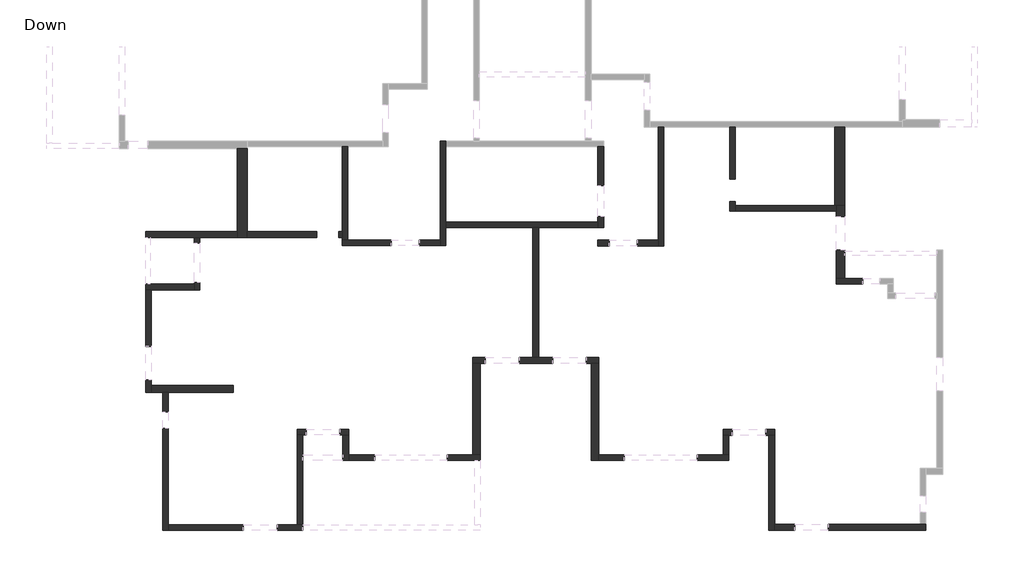
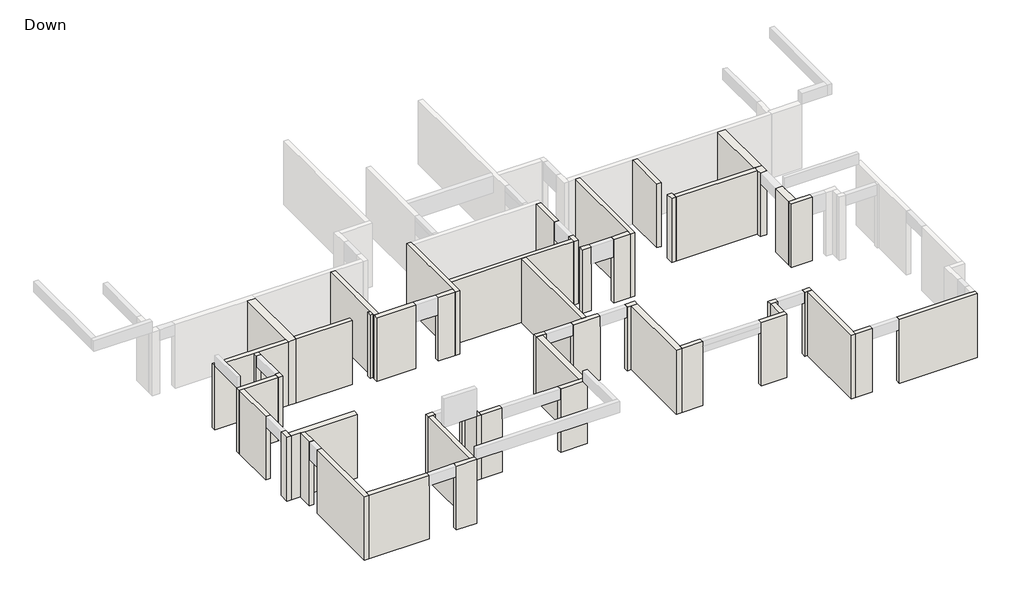
# One storey, part 1 of 3: 51 walls.
"""IFC4 building model written with IfcOpenShell, lengths in millimetres."""

from ifc_helpers import new_model, si_unit, origin, place, context, project, spatial, faceted_brep, element, save

model = new_model("IFC4")

# Units and contexts
model_context = context("Model", 3, world=origin())
ifc_project = project(units=[si_unit("LENGTHUNIT", "METRE", prefix="MILLI")], contexts=[model_context])

# Site, building, storey
site = spatial("IfcSite", under=ifc_project)
building = spatial("IfcBuilding", under=site)
storey = spatial("IfcBuildingStorey", under=building, Name="Down", Elevation=0.0)

# Walls
placement = place(None, origin())
element("IfcWall", 1, ObjectType="20", at=placement, inside=storey, context=model_context, shape_type="Brep", body=[
    faceted_brep([(-6090.9338154, -2994.7427075, 0.0), (-9365.9338154, -2994.7427075, 0.0), (-9365.9338154, -2994.7427075, 3000.0), (-6090.9338154, -2994.7427075, 3000.0), (-6090.9338154, -3194.7427075, 0.0), (-6090.9338154, -3194.7427075, 3000.0), (-7434.594706, -3194.7427075, 3000.0), (-7634.594706, -3194.7427075, 3000.0), (-9365.9338154, -3194.7427075, 3000.0), (-9365.9338154, -3194.7427075, 2780.0), (-9365.9338154, -3194.7427075, 0.0), (-7634.594706, -3194.7427075, 0.0), (-7434.594706, -3194.7427075, 0.0)], [[[0, 1, 2, 3]], [[4, 5, 6, 7, 8, 9, 10, 11, 12]], [[1, 0, 4, 12, 11, 10]], [[2, 1, 10, 9, 8]], [[3, 2, 8, 7, 6, 5]], [[0, 3, 5, 4]]]),
])
element("IfcWall", 2, ObjectType="20", at=placement, inside=storey, context=model_context, shape_type="Brep", body=[
    faceted_brep([(-7634.594706, -3194.7427075, 0.0), (-7634.594706, -3392.9835498, 0.0), (-7634.594706, -3392.9835498, 2500.0), (-7634.594706, -3392.9835498, 3000.0), (-7634.594706, -3194.7427075, 3000.0), (-7434.594706, -3194.7427075, 0.0), (-7434.594706, -3194.7427075, 2780.0), (-7434.594706, -3194.7427075, 3000.0), (-7434.594706, -3392.9835498, 3000.0), (-7434.594706, -3392.9835498, 2500.0), (-7434.594706, -3392.9835498, 0.0)], [[[0, 1, 2, 3, 4]], [[5, 6, 7, 8, 9, 10]], [[1, 0, 5, 10]], [[3, 2, 1, 10, 9, 8]], [[4, 3, 8, 7]], [[0, 4, 7, 6, 5]]]),
])
element("IfcWall", 3, ObjectType="20", at=placement, inside=storey, context=model_context, shape_type="Brep", body=[
    faceted_brep([(-5740.9338154, -3194.7427075, 0.0), (-3252.010806, -3194.7427075, 0.0), (-3252.010806, -3194.7427075, 2780.0), (-3252.010806, -3194.7427075, 3000.0), (-5740.9338154, -3194.7427075, 3000.0), (-5740.9338154, -2994.7427075, 0.0), (-5740.9338154, -2994.7427075, 2780.0), (-5740.9338154, -2994.7427075, 3000.0), (-3252.010806, -2994.7427075, 3000.0), (-3252.010806, -2994.7427075, 2780.0), (-3252.010806, -2994.7427075, 0.0)], [[[0, 1, 2, 3, 4]], [[5, 6, 7, 8, 9, 10]], [[1, 0, 5, 10]], [[3, 2, 1, 10, 9, 8]], [[4, 3, 8, 7]], [[0, 4, 7, 6, 5]]]),
])
element("IfcWall", 4, ObjectType="20", at=placement, inside=storey, context=model_context, shape_type="Brep", body=[
    faceted_brep([(-2456.1345173, -3194.0144776, 0.0), (-2336.5139865, -3194.0144776, 0.0), (-2336.5139865, -3194.0144776, 2780.0), (-2336.5139865, -3194.0144776, 3000.0), (-2456.1345173, -3194.0144776, 3000.0), (-2456.1345173, -3194.0144776, 2780.0), (-2456.1345173, -2994.0144776, 0.0), (-2456.1345173, -2994.0144776, 2780.0), (-2456.1345173, -2994.0144776, 3000.0), (-2336.5139865, -2994.0144776, 3000.0), (-2336.5139865, -2994.0144776, 2780.0), (-2336.5139865, -2994.0144776, 0.0), (-2456.1345173, -2994.7427075, 3000.0)], [[[0, 1, 2, 3, 4, 5]], [[6, 7, 8, 9, 10, 11]], [[1, 0, 6, 11]], [[4, 3, 9, 8, 12]], [[0, 5, 4, 12, 8, 7, 6]], [[3, 2, 1, 11, 10, 9]]]),
])
element("IfcWall", 5, ObjectType="20", at=placement, inside=storey, context=model_context, shape_type="Brep", body=[
    faceted_brep([(-2336.5139865, -3494.0144776, 0.0), (-591.3286388, -3494.0144776, 0.0), (-591.3286388, -3494.0144776, 2180.0), (-591.3286388, -3494.0144776, 3000.0), (-2336.5139865, -3494.0144776, 3000.0), (-2336.5139865, -3494.0144776, 2780.0), (-2336.5139865, -3294.0144776, 0.0), (-2336.5139865, -3294.0144776, 3000.0), (-2136.5139865, -3294.0144776, 3000.0), (-591.3286388, -3294.0144776, 3000.0), (-591.3286388, -3294.0144776, 2180.0), (-591.3286388, -3294.0144776, 0.0), (-2136.5139865, -3294.0144776, 0.0)], [[[0, 1, 2, 3, 4, 5]], [[6, 7, 8, 9, 10, 11, 12]], [[1, 0, 6, 12, 11]], [[3, 2, 1, 11, 10, 9]], [[4, 3, 9, 8, 7]], [[0, 5, 4, 7, 6]]]),
])
element("IfcWall", 6, ObjectType="20", at=placement, inside=storey, context=model_context, shape_type="Brep", body=[
    faceted_brep([(-2136.5139865, -3294.0144776, 0.0), (-2136.5139865, 51.1884177, 0.0), (-2136.5139865, 51.1884177, 2780.0), (-2136.5139865, 51.1884177, 3000.0), (-2136.5139865, -3294.0144776, 3000.0), (-2136.5139865, -3294.0144776, 2780.0), (-2336.5139865, -3294.0144776, 0.0), (-2336.5139865, -3294.0144776, 3000.0), (-2336.5139865, -3194.0144776, 3000.0), (-2336.5139865, -2994.0144776, 3000.0), (-2336.5139865, 51.1884177, 3000.0), (-2336.5139865, 51.1884177, 2780.0), (-2336.5139865, 51.1884177, 0.0), (-2336.5139865, -2994.0144776, 0.0), (-2336.5139865, -3194.0144776, 0.0)], [[[0, 1, 2, 3, 4, 5]], [[6, 7, 8, 9, 10, 11, 12, 13, 14]], [[1, 0, 6, 14, 13, 12]], [[4, 3, 10, 9, 8, 7]], [[3, 2, 1, 12, 11, 10]], [[0, 5, 4, 7, 6]]]),
])
element("IfcWall", 7, ObjectType="20", at=placement, inside=storey, context=model_context, shape_type="Brep", body=[
    faceted_brep([(1160.820407, 252.3535615, 0.0), (1160.820407, -3294.0144776, 0.0), (1160.820407, -3494.0144776, 0.0), (1160.820407, -3494.0144776, 3000.0), (1160.820407, -3294.0144776, 3000.0), (1160.820407, 252.3535615, 3000.0), (1160.820407, 252.3535615, 2780.0), (1360.820407, 252.3535615, 0.0), (1360.820407, 252.3535615, 3000.0), (1360.820407, 52.3535615, 3000.0), (1360.820407, -2647.6464385, 3000.0), (1360.820407, -2847.6464385, 3000.0), (1360.820407, -3494.0144776, 3000.0), (1360.820407, -3494.0144776, 2780.0), (1360.820407, -3494.0144776, 0.0), (1360.820407, -2847.6464385, 0.0), (1360.820407, -2647.6464385, 0.0), (1360.820407, 52.3535615, 0.0)], [[[0, 1, 2, 3, 4, 5, 6]], [[7, 8, 9, 10, 11, 12, 13, 14, 15, 16, 17]], [[2, 1, 0, 7, 17, 16, 15, 14]], [[5, 4, 3, 12, 11, 10, 9, 8]], [[3, 2, 14, 13, 12]], [[0, 6, 5, 8, 7]]]),
])
element("IfcWall", 8, ObjectType="20", at=placement, inside=storey, context=model_context, shape_type="Brep", body=[
    faceted_brep([(1360.820407, -2847.6464385, 0.0), (4485.405294, -2847.6464385, 0.0), (4685.405294, -2847.6464385, 0.0), (6810.820407, -2847.6464385, 0.0), (6810.820407, -2847.6464385, 2780.0), (6810.820407, -2847.6464385, 3000.0), (4685.405294, -2847.6464385, 3000.0), (4485.405294, -2847.6464385, 3000.0), (1360.820407, -2847.6464385, 3000.0), (1360.820407, -2847.6464385, 2780.0), (1360.820407, -2647.6464385, 0.0), (1360.820407, -2647.6464385, 3000.0), (6810.820407, -2647.6464385, 3000.0), (6810.820407, -2647.6464385, 0.0)], [[[0, 1, 2, 3, 4, 5, 6, 7, 8, 9]], [[10, 11, 12, 13]], [[3, 2, 1, 0, 10, 13]], [[8, 7, 6, 5, 12, 11]], [[0, 9, 8, 11, 10]], [[5, 4, 3, 13, 12]]]),
])
element("IfcWall", 9, ObjectType="20", at=placement, inside=storey, context=model_context, shape_type="Brep", body=[
    faceted_brep([(7010.820407, -2847.6464385, 0.0), (7010.820407, -2447.6464385, 0.0), (7010.820407, -2447.6464385, 2180.0), (7010.820407, -2447.6464385, 3000.0), (7010.820407, -2847.6464385, 3000.0), (7010.820407, -2847.6464385, 2780.0), (6810.820407, -2847.6464385, 0.0), (6810.820407, -2847.6464385, 2780.0), (6810.820407, -2847.6464385, 3000.0), (6810.820407, -2647.6464385, 3000.0), (6810.820407, -2447.6464385, 3000.0), (6810.820407, -2447.6464385, 2180.0), (6810.820407, -2447.6464385, 0.0), (6810.820407, -2647.6464385, 0.0)], [[[0, 1, 2, 3, 4, 5]], [[6, 7, 8, 9, 10, 11, 12, 13]], [[1, 0, 6, 13, 12]], [[3, 2, 1, 12, 11, 10]], [[4, 3, 10, 9, 8]], [[0, 5, 4, 8, 7, 6]]]),
])
element("IfcWall", 10, ObjectType="20", at=placement, inside=storey, context=model_context, shape_type="Brep", body=[
    faceted_brep([(6810.820407, 52.3535615, 0.0), (6810.820407, -1347.6464385, 0.0), (6810.820407, -1347.6464385, 2180.0), (6810.820407, -1347.6464385, 3000.0), (6810.820407, 52.3535615, 3000.0), (7010.820407, 52.3535615, 0.0), (7010.820407, 52.3535615, 3000.0), (7010.820407, -1347.6464385, 3000.0), (7010.820407, -1347.6464385, 2180.0), (7010.820407, -1347.6464385, 0.0)], [[[0, 1, 2, 3, 4]], [[5, 6, 7, 8, 9]], [[1, 0, 5, 9]], [[3, 2, 1, 9, 8, 7]], [[4, 3, 7, 6]], [[0, 4, 6, 5]]]),
])
element("IfcWall", 11, ObjectType="20", at=placement, inside=storey, context=model_context, shape_type="Brep", body=[
    faceted_brep([(-7634.594706, -4812.9835498, 0.0), (-7634.594706, -4872.9835498, 0.0), (-7634.594706, -5072.9835498, 0.0), (-7634.594706, -5072.9835498, 3000.0), (-7634.594706, -4872.9835498, 3000.0), (-7634.594706, -4812.9835498, 3000.0), (-7634.594706, -4812.9835498, 2500.0), (-7434.594706, -4812.9835498, 0.0), (-7434.594706, -4812.9835498, 2500.0), (-7434.594706, -4812.9835498, 3000.0), (-7434.594706, -5072.9835498, 3000.0), (-7434.594706, -5072.9835498, 2780.0), (-7434.594706, -5072.9835498, 0.0)], [[[0, 1, 2, 3, 4, 5, 6]], [[7, 8, 9, 10, 11, 12]], [[2, 1, 0, 7, 12]], [[5, 4, 3, 10, 9]], [[0, 6, 5, 9, 8, 7]], [[3, 2, 12, 11, 10]]]),
])
element("IfcWall", 12, ObjectType="20", at=placement, inside=storey, context=model_context, shape_type="Brep", body=[
    faceted_brep([(-7634.594706, -4872.9835498, 0.0), (-9364.594706, -4872.9835498, 0.0), (-9364.594706, -4872.9835498, 3000.0), (-7634.594706, -4872.9835498, 3000.0), (-7634.594706, -4872.9835498, 2780.0), (-7634.594706, -5072.9835498, 0.0), (-7634.594706, -5072.9835498, 3000.0), (-9164.594706, -5072.9835498, 3000.0), (-9364.594706, -5072.9835498, 3000.0), (-9364.594706, -5072.9835498, 0.0), (-9164.594706, -5072.9835498, 0.0)], [[[0, 1, 2, 3, 4]], [[5, 6, 7, 8, 9, 10]], [[1, 0, 5, 10, 9]], [[3, 2, 8, 7, 6]], [[0, 4, 3, 6, 5]], [[2, 1, 9, 8]]]),
])
element("IfcWall", 13, ObjectType="20", at=placement, inside=storey, context=model_context, shape_type="Brep", body=[
    faceted_brep([(-9364.594706, -5072.9835498, 0.0), (-9364.594706, -7092.9835498, 0.0), (-9364.594706, -7092.9835498, 2500.0), (-9364.594706, -7092.9835498, 3000.0), (-9364.594706, -5072.9835498, 3000.0), (-9164.594706, -5072.9835498, 0.0), (-9164.594706, -5072.9835498, 2780.0), (-9164.594706, -5072.9835498, 3000.0), (-9164.594706, -7092.9835498, 3000.0), (-9164.594706, -7092.9835498, 2500.0), (-9164.594706, -7092.9835498, 0.0)], [[[0, 1, 2, 3, 4]], [[5, 6, 7, 8, 9, 10]], [[1, 0, 5, 10]], [[3, 2, 1, 10, 9, 8]], [[4, 3, 8, 7]], [[0, 4, 7, 6, 5]]]),
])
element("IfcWall", 14, ObjectType="20", at=placement, inside=storey, context=model_context, shape_type="Brep", body=[
    faceted_brep([(-9364.594706, -8292.9835498, 0.0), (-9364.594706, -8747.9835498, 0.0), (-9364.594706, -8747.9835498, 3000.0), (-9364.594706, -8292.9835498, 3000.0), (-9364.594706, -8292.9835498, 2500.0), (-9164.594706, -8292.9835498, 0.0), (-9164.594706, -8292.9835498, 2500.0), (-9164.594706, -8292.9835498, 3000.0), (-9164.594706, -8497.9835498, 3000.0), (-9164.594706, -8747.9835498, 3000.0), (-9164.594706, -8747.9835498, 0.0), (-9164.594706, -8497.9835498, 0.0)], [[[0, 1, 2, 3, 4]], [[5, 6, 7, 8, 9, 10, 11]], [[1, 0, 5, 11, 10]], [[3, 2, 9, 8, 7]], [[0, 4, 3, 7, 6, 5]], [[2, 1, 10, 9]]]),
])
element("IfcWall", 15, ObjectType="20", at=placement, inside=storey, context=model_context, shape_type="Brep", body=[
    faceted_brep([(-8764.594706, -8747.9835498, 0.0), (-8764.594706, -9442.9835498, 0.0), (-8764.594706, -9442.9835498, 2180.0), (-8764.594706, -9442.9835498, 3000.0), (-8764.594706, -8747.9835498, 3000.0), (-8564.594706, -8747.9835498, 0.0), (-8564.594706, -8747.9835498, 2780.0), (-8564.594706, -8747.9835498, 3000.0), (-8564.594706, -9442.9835498, 3000.0), (-8564.594706, -9442.9835498, 2180.0), (-8564.594706, -9442.9835498, 0.0)], [[[0, 1, 2, 3, 4]], [[5, 6, 7, 8, 9, 10]], [[1, 0, 5, 10]], [[3, 2, 1, 10, 9, 8]], [[4, 3, 8, 7]], [[0, 4, 7, 6, 5]]]),
])
element("IfcWall", 16, ObjectType="20", at=placement, inside=storey, context=model_context, shape_type="Brep", body=[
    faceted_brep([(-8764.594706, -10042.9835498, 0.0), (-8764.594706, -13682.9835498, 0.0), (-8764.594706, -13682.9835498, 3000.0), (-8764.594706, -10042.9835498, 3000.0), (-8764.594706, -10042.9835498, 2180.0), (-8564.594706, -10042.9835498, 0.0), (-8564.594706, -10042.9835498, 2180.0), (-8564.594706, -10042.9835498, 3000.0), (-8564.594706, -13482.9835498, 3000.0), (-8564.594706, -13682.9835498, 3000.0), (-8564.594706, -13682.9835498, 0.0), (-8564.594706, -13482.9835498, 0.0)], [[[0, 1, 2, 3, 4]], [[5, 6, 7, 8, 9, 10, 11]], [[1, 0, 5, 11, 10]], [[3, 2, 9, 8, 7]], [[0, 4, 3, 7, 6, 5]], [[2, 1, 10, 9]]]),
])
element("IfcWall", 17, ObjectType="20", at=placement, inside=storey, context=model_context, shape_type="Brep", body=[
    faceted_brep([(-8564.594706, -13682.9835498, 0.0), (-5884.594706, -13682.9835498, 0.0), (-5884.594706, -13682.9835498, 2500.0), (-5884.594706, -13682.9835498, 3000.0), (-8564.594706, -13682.9835498, 3000.0), (-8564.594706, -13482.9835498, 0.0), (-8564.594706, -13482.9835498, 2780.0), (-8564.594706, -13482.9835498, 3000.0), (-5884.594706, -13482.9835498, 3000.0), (-5884.594706, -13482.9835498, 2500.0), (-5884.594706, -13482.9835498, 0.0)], [[[0, 1, 2, 3, 4]], [[5, 6, 7, 8, 9, 10]], [[1, 0, 5, 10]], [[3, 2, 1, 10, 9, 8]], [[4, 3, 8, 7]], [[0, 4, 7, 6, 5]]]),
])
element("IfcWall", 18, ObjectType="20", at=placement, inside=storey, context=model_context, shape_type="Brep", body=[
    faceted_brep([(-4664.594706, -13682.9835498, 0.0), (-3754.594706, -13682.9835498, 0.0), (-3754.594706, -13682.9835498, 3000.0), (-4664.594706, -13682.9835498, 3000.0), (-4664.594706, -13682.9835498, 2500.0), (-4664.594706, -13482.9835498, 0.0), (-4664.594706, -13482.9835498, 2500.0), (-4664.594706, -13482.9835498, 3000.0), (-3954.594706, -13482.9835498, 3000.0), (-3754.594706, -13482.9835498, 3000.0), (-3754.594706, -13482.9835498, 0.0), (-3954.594706, -13482.9835498, 0.0)], [[[0, 1, 2, 3, 4]], [[5, 6, 7, 8, 9, 10, 11]], [[1, 0, 5, 11, 10]], [[3, 2, 9, 8, 7]], [[0, 4, 3, 7, 6, 5]], [[2, 1, 10, 9]]]),
])
element("IfcWall", 19, ObjectType="20", at=placement, inside=storey, context=model_context, shape_type="Brep", body=[
    faceted_brep([(-3754.594706, -13482.9835498, 0.0), (-3754.594706, -10272.9835498, 0.0), (-3754.594706, -10272.9835498, 3000.0), (-3754.594706, -10977.9835498, 3000.0), (-3754.594706, -13482.9835498, 3000.0), (-3954.594706, -13482.9835498, 0.0), (-3954.594706, -13482.9835498, 2780.0), (-3954.594706, -13482.9835498, 3000.0), (-3954.594706, -10272.9835498, 3000.0), (-3954.594706, -10272.9835498, 0.0)], [[[0, 1, 2, 3, 4]], [[5, 6, 7, 8, 9]], [[1, 0, 5, 9]], [[4, 3, 2, 8, 7]], [[0, 4, 7, 6, 5]], [[2, 1, 9, 8]]]),
])
element("IfcWall", 20, ObjectType="20", at=placement, inside=storey, context=model_context, shape_type="Brep", body=[
    faceted_brep([(-3954.594706, -10272.9835498, 0.0), (-3754.594706, -10272.9835498, 0.0), (-3634.594706, -10272.9835498, 0.0), (-3634.594706, -10272.9835498, 2500.0), (-3634.594706, -10272.9835498, 3000.0), (-3754.594706, -10272.9835498, 3000.0), (-3954.594706, -10272.9835498, 3000.0), (-3954.594706, -10072.9835498, 0.0), (-3954.594706, -10072.9835498, 2780.0), (-3954.594706, -10072.9835498, 3000.0), (-3634.594706, -10072.9835498, 3000.0), (-3634.594706, -10072.9835498, 2500.0), (-3634.594706, -10072.9835498, 0.0)], [[[0, 1, 2, 3, 4, 5, 6]], [[7, 8, 9, 10, 11, 12]], [[2, 1, 0, 7, 12]], [[4, 3, 2, 12, 11, 10]], [[6, 5, 4, 10, 9]], [[0, 6, 9, 8, 7]]]),
])
element("IfcWall", 21, ObjectType="20", at=placement, inside=storey, context=model_context, shape_type="Brep", body=[
    faceted_brep([(-2434.594706, -10272.9835498, 0.0), (-2314.594706, -10272.9835498, 0.0), (-2114.594706, -10272.9835498, 0.0), (-2114.594706, -10272.9835498, 3000.0), (-2314.594706, -10272.9835498, 3000.0), (-2434.594706, -10272.9835498, 3000.0), (-2434.594706, -10272.9835498, 2500.0), (-2434.594706, -10072.9835498, 0.0), (-2434.594706, -10072.9835498, 2500.0), (-2434.594706, -10072.9835498, 3000.0), (-2114.594706, -10072.9835498, 3000.0), (-2114.594706, -10072.9835498, 2780.0), (-2114.594706, -10072.9835498, 0.0)], [[[0, 1, 2, 3, 4, 5, 6]], [[7, 8, 9, 10, 11, 12]], [[2, 1, 0, 7, 12]], [[5, 4, 3, 10, 9]], [[0, 6, 5, 9, 8, 7]], [[3, 2, 12, 11, 10]]]),
])
element("IfcWall", 22, ObjectType="20", at=placement, inside=storey, context=model_context, shape_type="Brep", body=[
    faceted_brep([(-2314.594706, -10272.9835498, 0.0), (-2314.594706, -11177.9835498, 0.0), (-2314.594706, -11177.9835498, 2780.0), (-2314.594706, -11177.9835498, 3000.0), (-2314.594706, -10977.9835498, 3000.0), (-2314.594706, -10272.9835498, 3000.0), (-2114.594706, -10272.9835498, 0.0), (-2114.594706, -10272.9835498, 3000.0), (-2114.594706, -10977.9835498, 3000.0), (-2114.594706, -11177.9835498, 3000.0), (-2114.594706, -11177.9835498, 0.0), (-2114.594706, -10977.9835498, 0.0)], [[[0, 1, 2, 3, 4, 5]], [[6, 7, 8, 9, 10, 11]], [[1, 0, 6, 11, 10]], [[5, 4, 3, 9, 8, 7]], [[0, 5, 7, 6]], [[3, 2, 1, 10, 9]]]),
])
element("IfcWall", 23, ObjectType="20", at=placement, inside=storey, context=model_context, shape_type="Brep", body=[
    faceted_brep([(-2114.594706, -11177.9835498, 0.0), (-1184.594706, -11177.9835498, 0.0), (-1184.594706, -11177.9835498, 2500.0), (-1184.594706, -11177.9835498, 3000.0), (-2114.594706, -11177.9835498, 3000.0), (-2114.594706, -10977.9835498, 0.0), (-2114.594706, -10977.9835498, 2780.0), (-2114.594706, -10977.9835498, 3000.0), (-1184.594706, -10977.9835498, 3000.0), (-1184.594706, -10977.9835498, 2500.0), (-1184.594706, -10977.9835498, 0.0)], [[[0, 1, 2, 3, 4]], [[5, 6, 7, 8, 9, 10]], [[1, 0, 5, 10]], [[3, 2, 1, 10, 9, 8]], [[4, 3, 8, 7]], [[0, 4, 7, 6, 5]]]),
])
element("IfcWall", 24, ObjectType="20", at=placement, inside=storey, context=model_context, shape_type="Brep", body=[
    faceted_brep([(1415.405294, -11177.9835498, 0.0), (2605.405294, -11177.9835498, 0.0), (2605.405294, -11177.9835498, 2780.0), (2605.405294, -11177.9835498, 3000.0), (1415.405294, -11177.9835498, 3000.0), (1415.405294, -11177.9835498, 2500.0), (1415.405294, -10977.9835498, 0.0), (1415.405294, -10977.9835498, 2500.0), (1415.405294, -10977.9835498, 3000.0), (2335.405294, -10977.9835498, 3000.0), (2605.405294, -10977.9835498, 3000.0), (2605.405294, -10977.9835498, 0.0), (2335.405294, -10977.9835498, 0.0)], [[[0, 1, 2, 3, 4, 5]], [[6, 7, 8, 9, 10, 11, 12]], [[1, 0, 6, 12, 11]], [[4, 3, 10, 9, 8]], [[0, 5, 4, 8, 7, 6]], [[3, 2, 1, 11, 10]]]),
])
element("IfcWall", 25, ObjectType="20", at=placement, inside=storey, context=model_context, shape_type="Brep", body=[
    faceted_brep([(2335.405294, -7702.9835498, 0.0), (2605.405294, -7702.9835498, 0.0), (2785.405294, -7702.9835498, 0.0), (2785.405294, -7702.9835498, 2500.0), (2785.405294, -7702.9835498, 3000.0), (2605.405294, -7702.9835498, 3000.0), (2335.405294, -7702.9835498, 3000.0), (2335.405294, -7502.9835498, 0.0), (2335.405294, -7502.9835498, 2780.0), (2335.405294, -7502.9835498, 3000.0), (2785.405294, -7502.9835498, 3000.0), (2785.405294, -7502.9835498, 2500.0), (2785.405294, -7502.9835498, 0.0)], [[[0, 1, 2, 3, 4, 5, 6]], [[7, 8, 9, 10, 11, 12]], [[2, 1, 0, 7, 12]], [[4, 3, 2, 12, 11, 10]], [[6, 5, 4, 10, 9]], [[0, 6, 9, 8, 7]]]),
])
element("IfcWall", 26, ObjectType="20", at=placement, inside=storey, context=model_context, shape_type="Brep", body=[
    faceted_brep([(3985.405294, -7702.9835498, 0.0), (5185.405294, -7702.9835498, 0.0), (5185.405294, -7702.9835498, 2500.0), (5185.405294, -7702.9835498, 3000.0), (3985.405294, -7702.9835498, 3000.0), (3985.405294, -7702.9835498, 2500.0), (3985.405294, -7502.9835498, 0.0), (3985.405294, -7502.9835498, 2500.0), (3985.405294, -7502.9835498, 3000.0), (4485.405294, -7502.9835498, 3000.0), (4685.405294, -7502.9835498, 3000.0), (5185.405294, -7502.9835498, 3000.0), (5185.405294, -7502.9835498, 2500.0), (5185.405294, -7502.9835498, 0.0), (4685.405294, -7502.9835498, 0.0), (4485.405294, -7502.9835498, 0.0)], [[[0, 1, 2, 3, 4, 5]], [[6, 7, 8, 9, 10, 11, 12, 13, 14, 15]], [[1, 0, 6, 15, 14, 13]], [[3, 2, 1, 13, 12, 11]], [[4, 3, 11, 10, 9, 8]], [[0, 5, 4, 8, 7, 6]]]),
])
element("IfcWall", 27, ObjectType="20", at=placement, inside=storey, context=model_context, shape_type="Brep", body=[
    faceted_brep([(6385.405294, -7702.9835498, 0.0), (6565.405294, -7702.9835498, 0.0), (6835.405294, -7702.9835498, 0.0), (6835.405294, -7702.9835498, 3000.0), (6565.405294, -7702.9835498, 3000.0), (6385.405294, -7702.9835498, 3000.0), (6385.405294, -7702.9835498, 2500.0), (6385.405294, -7502.9835498, 0.0), (6385.405294, -7502.9835498, 2500.0), (6385.405294, -7502.9835498, 3000.0), (6835.405294, -7502.9835498, 3000.0), (6835.405294, -7502.9835498, 2780.0), (6835.405294, -7502.9835498, 0.0)], [[[0, 1, 2, 3, 4, 5, 6]], [[7, 8, 9, 10, 11, 12]], [[2, 1, 0, 7, 12]], [[5, 4, 3, 10, 9]], [[0, 6, 5, 9, 8, 7]], [[3, 2, 12, 11, 10]]]),
])
element("IfcWall", 28, ObjectType="20", at=placement, inside=storey, context=model_context, shape_type="Brep", body=[
    faceted_brep([(4685.405294, -7502.9835498, 0.0), (4685.405294, -2847.6464385, 0.0), (4685.405294, -2847.6464385, 2780.0), (4685.405294, -2847.6464385, 3000.0), (4685.405294, -7502.9835498, 3000.0), (4685.405294, -7502.9835498, 2780.0), (4485.405294, -7502.9835498, 0.0), (4485.405294, -7502.9835498, 2780.0), (4485.405294, -7502.9835498, 3000.0), (4485.405294, -2847.6464385, 3000.0), (4485.405294, -2847.6464385, 2780.0), (4485.405294, -2847.6464385, 0.0)], [[[0, 1, 2, 3, 4, 5]], [[6, 7, 8, 9, 10, 11]], [[1, 0, 6, 11]], [[4, 3, 9, 8]], [[3, 2, 1, 11, 10, 9]], [[0, 5, 4, 8, 7, 6]]]),
])
element("IfcWall", 29, ObjectType="20", at=placement, inside=storey, context=model_context, shape_type="Brep", body=[
    faceted_brep([(6835.405294, -11177.9835498, 0.0), (7755.405294, -11177.9835498, 0.0), (7755.405294, -11177.9835498, 2500.0), (7755.405294, -11177.9835498, 2780.0), (7755.405294, -11177.9835498, 3000.0), (6835.405294, -11177.9835498, 3000.0), (6835.405294, -10977.9835498, 0.0), (6835.405294, -10977.9835498, 2780.0), (6835.405294, -10977.9835498, 3000.0), (7755.405294, -10977.9835498, 3000.0), (7755.405294, -10977.9835498, 2500.0), (7755.405294, -10977.9835498, 0.0), (7755.405294, -11172.9835498, 3000.0)], [[[0, 1, 2, 3, 4, 5]], [[6, 7, 8, 9, 10, 11]], [[1, 0, 6, 11]], [[4, 3, 2, 1, 11, 10, 9, 12]], [[5, 4, 12, 9, 8]], [[0, 5, 8, 7, 6]]]),
])
element("IfcWall", 30, ObjectType="20", at=placement, inside=storey, context=model_context, shape_type="Brep", body=[
    faceted_brep([(10357.905294, -11177.9835498, 0.0), (11487.905294, -11177.9835498, 0.0), (11487.905294, -11177.9835498, 2780.0), (11487.905294, -11177.9835498, 3000.0), (10357.905294, -11177.9835498, 3000.0), (10357.905294, -11177.9835498, 2780.0), (10357.905294, -11177.9835498, 2500.0), (10357.905294, -10977.9835498, 0.0), (10357.905294, -10977.9835498, 2500.0), (10357.905294, -10977.9835498, 3000.0), (11287.905294, -10977.9835498, 3000.0), (11487.905294, -10977.9835498, 3000.0), (11487.905294, -10977.9835498, 0.0), (11287.905294, -10977.9835498, 0.0), (10357.905294, -11172.9835498, 3000.0)], [[[0, 1, 2, 3, 4, 5, 6]], [[7, 8, 9, 10, 11, 12, 13]], [[1, 0, 7, 13, 12]], [[4, 3, 11, 10, 9, 14]], [[0, 6, 5, 4, 14, 9, 8, 7]], [[3, 2, 1, 12, 11]]]),
])
element("IfcWall", 31, ObjectType="20", at=placement, inside=storey, context=model_context, shape_type="Brep", body=[
    faceted_brep([(11487.905294, -10977.9835498, 0.0), (11487.905294, -10277.9835498, 0.0), (11487.905294, -10277.9835498, 3000.0), (11487.905294, -10972.9835498, 3000.0), (11487.905294, -10977.9835498, 3000.0), (11287.905294, -10977.9835498, 0.0), (11287.905294, -10977.9835498, 2780.0), (11287.905294, -10977.9835498, 3000.0), (11287.905294, -10277.9835498, 3000.0), (11287.905294, -10277.9835498, 0.0)], [[[0, 1, 2, 3, 4]], [[5, 6, 7, 8, 9]], [[1, 0, 5, 9]], [[4, 3, 2, 8, 7]], [[0, 4, 7, 6, 5]], [[2, 1, 9, 8]]]),
])
element("IfcWall", 32, ObjectType="20", at=placement, inside=storey, context=model_context, shape_type="Brep", body=[
    faceted_brep([(11287.905294, -10277.9835498, 0.0), (11487.905294, -10277.9835498, 0.0), (11607.905294, -10277.9835498, 0.0), (11607.905294, -10277.9835498, 2500.0), (11607.905294, -10277.9835498, 3000.0), (11487.905294, -10277.9835498, 3000.0), (11287.905294, -10277.9835498, 3000.0), (11287.905294, -10077.9835498, 0.0), (11287.905294, -10077.9835498, 2780.0), (11287.905294, -10077.9835498, 3000.0), (11607.905294, -10077.9835498, 3000.0), (11607.905294, -10077.9835498, 2500.0), (11607.905294, -10077.9835498, 0.0)], [[[0, 1, 2, 3, 4, 5, 6]], [[7, 8, 9, 10, 11, 12]], [[2, 1, 0, 7, 12]], [[4, 3, 2, 12, 11, 10]], [[6, 5, 4, 10, 9]], [[0, 6, 9, 8, 7]]]),
])
element("IfcWall", 33, ObjectType="20", at=placement, inside=storey, context=model_context, shape_type="Brep", body=[
    faceted_brep([(12807.905294, -10277.9835498, 0.0), (12927.905294, -10277.9835498, 0.0), (13127.905294, -10277.9835498, 0.0), (13127.905294, -10277.9835498, 3000.0), (12927.905294, -10277.9835498, 3000.0), (12807.905294, -10277.9835498, 3000.0), (12807.905294, -10277.9835498, 2500.0), (12807.905294, -10077.9835498, 0.0), (12807.905294, -10077.9835498, 2500.0), (12807.905294, -10077.9835498, 3000.0), (13127.905294, -10077.9835498, 3000.0), (13127.905294, -10077.9835498, 2780.0), (13127.905294, -10077.9835498, 0.0)], [[[0, 1, 2, 3, 4, 5, 6]], [[7, 8, 9, 10, 11, 12]], [[2, 1, 0, 7, 12]], [[5, 4, 3, 10, 9]], [[0, 6, 5, 9, 8, 7]], [[3, 2, 12, 11, 10]]]),
])
element("IfcWall", 34, ObjectType="20", at=placement, inside=storey, context=model_context, shape_type="Brep", body=[
    faceted_brep([(12927.905294, -10277.9835498, 0.0), (12927.905294, -13677.9835498, 0.0), (12927.905294, -13677.9835498, 2780.0), (12927.905294, -13677.9835498, 3000.0), (12927.905294, -10972.9835498, 3000.0), (12927.905294, -10277.9835498, 3000.0), (13127.905294, -10277.9835498, 0.0), (13127.905294, -10277.9835498, 3000.0), (13127.905294, -13477.9835498, 3000.0), (13127.905294, -13677.9835498, 3000.0), (13127.905294, -13677.9835498, 0.0), (13127.905294, -13477.9835498, 0.0)], [[[0, 1, 2, 3, 4, 5]], [[6, 7, 8, 9, 10, 11]], [[1, 0, 6, 11, 10]], [[5, 4, 3, 9, 8, 7]], [[0, 5, 7, 6]], [[3, 2, 1, 10, 9]]]),
])
element("IfcWall", 35, ObjectType="20", at=placement, inside=storey, context=model_context, shape_type="Brep", body=[
    faceted_brep([(13127.905294, -13677.9835498, 0.0), (13857.905294, -13677.9835498, 0.0), (13857.905294, -13677.9835498, 2500.0), (13857.905294, -13677.9835498, 3000.0), (13127.905294, -13677.9835498, 3000.0), (13127.905294, -13477.9835498, 0.0), (13127.905294, -13477.9835498, 2780.0), (13127.905294, -13477.9835498, 3000.0), (13857.905294, -13477.9835498, 3000.0), (13857.905294, -13477.9835498, 2500.0), (13857.905294, -13477.9835498, 0.0)], [[[0, 1, 2, 3, 4]], [[5, 6, 7, 8, 9, 10]], [[1, 0, 5, 10]], [[3, 2, 1, 10, 9, 8]], [[4, 3, 8, 7]], [[0, 4, 7, 6, 5]]]),
])
element("IfcWall", 36, ObjectType="20", at=placement, inside=storey, context=model_context, shape_type="Brep", body=[
    faceted_brep([(15057.905294, -13677.9835498, 0.0), (18537.905294, -13677.9835498, 0.0), (18537.905294, -13677.9835498, 3000.0), (15057.905294, -13677.9835498, 3000.0), (15057.905294, -13677.9835498, 2500.0), (15057.905294, -13477.9835498, 0.0), (15057.905294, -13477.9835498, 2500.0), (15057.905294, -13477.9835498, 3000.0), (18337.905294, -13477.9835498, 3000.0), (18537.905294, -13477.9835498, 3000.0), (18537.905294, -13477.9835498, 0.0), (18337.905294, -13477.9835498, 0.0)], [[[0, 1, 2, 3, 4]], [[5, 6, 7, 8, 9, 10, 11]], [[1, 0, 5, 11, 10]], [[3, 2, 9, 8, 7]], [[0, 4, 3, 7, 6, 5]], [[2, 1, 10, 9]]]),
])
element("IfcWall", 37, ObjectType="20", at=placement, inside=storey, context=model_context, shape_type="Brep", body=[
    faceted_brep([(16277.905294, -4662.9835498, 0.0), (15639.9526685, -4662.9835498, 0.0), (15339.9526685, -4662.9835498, 0.0), (15339.9526685, -4662.9835498, 3000.0), (15639.9526685, -4662.9835498, 3000.0), (16277.905294, -4662.9835498, 3000.0), (16277.905294, -4662.9835498, 2180.0), (16277.905294, -4862.9835498, 0.0), (16277.905294, -4862.9835498, 2180.0), (16277.905294, -4862.9835498, 3000.0), (15339.9526685, -4862.9835498, 3000.0), (15339.9526685, -4862.9835498, 2780.0), (15339.9526685, -4862.9835498, 0.0)], [[[0, 1, 2, 3, 4, 5, 6]], [[7, 8, 9, 10, 11, 12]], [[2, 1, 0, 7, 12]], [[5, 4, 3, 10, 9]], [[0, 6, 5, 9, 8, 7]], [[3, 2, 12, 11, 10]]]),
])
element("IfcWall", 38, ObjectType="20", at=placement, inside=storey, context=model_context, shape_type="Brep", body=[
    faceted_brep([(15339.9526685, -2047.9835498, 0.0), (15289.9526685, -2047.9835498, 0.0), (11717.905294, -2047.9835498, 0.0), (11717.905294, -2047.9835498, 2780.0), (11717.905294, -2047.9835498, 3000.0), (15289.9526685, -2047.9835498, 3000.0), (15339.9526685, -2047.9835498, 3000.0), (15339.9526685, -2247.9835498, 0.0), (15339.9526685, -2247.9835498, 2780.0), (15339.9526685, -2247.9835498, 3000.0), (11717.905294, -2247.9835498, 3000.0), (11717.905294, -2247.9835498, 0.0)], [[[0, 1, 2, 3, 4, 5, 6]], [[7, 8, 9, 10, 11]], [[2, 1, 0, 7, 11]], [[6, 5, 4, 10, 9]], [[0, 6, 9, 8, 7]], [[4, 3, 2, 11, 10]]]),
])
element("IfcWall", 39, ObjectType="20", at=placement, inside=storey, context=model_context, shape_type="Brep", body=[
    faceted_brep([(11717.905294, -2247.9835498, 0.0), (11717.905294, -2047.9835498, 0.0), (11717.905294, -1907.9835498, 0.0), (11717.905294, -1907.9835498, 2780.0), (11717.905294, -1907.9835498, 3000.0), (11717.905294, -2047.9835498, 3000.0), (11717.905294, -2247.9835498, 3000.0), (11517.905294, -2247.9835498, 0.0), (11517.905294, -2247.9835498, 2780.0), (11517.905294, -2247.9835498, 3000.0), (11517.905294, -1907.9835498, 3000.0), (11517.905294, -1907.9835498, 2780.0), (11517.905294, -1907.9835498, 0.0)], [[[0, 1, 2, 3, 4, 5, 6]], [[7, 8, 9, 10, 11, 12]], [[2, 1, 0, 7, 12]], [[4, 3, 2, 12, 11, 10]], [[6, 5, 4, 10, 9]], [[0, 6, 9, 8, 7]]]),
])
element("IfcWall", 40, ObjectType="20", at=placement, inside=storey, context=model_context, shape_type="Brep", body=[
    faceted_brep([(11717.905294, -1107.9835498, 0.0), (11717.905294, 752.0164502, 0.0), (11717.905294, 752.0164502, 2780.0), (11717.905294, 752.0164502, 3000.0), (11717.905294, -1107.9835498, 3000.0), (11717.905294, -1107.9835498, 2780.0), (11517.905294, -1107.9835498, 0.0), (11517.905294, -1107.9835498, 2780.0), (11517.905294, -1107.9835498, 3000.0), (11517.905294, 752.0164502, 3000.0), (11517.905294, 752.0164502, 2780.0), (11517.905294, 752.0164502, 0.0)], [[[0, 1, 2, 3, 4, 5]], [[6, 7, 8, 9, 10, 11]], [[1, 0, 6, 11]], [[4, 3, 9, 8]], [[0, 5, 4, 8, 7, 6]], [[3, 2, 1, 11, 10, 9]]]),
])
element("IfcWall", 41, ObjectType="20", at=placement, inside=storey, context=model_context, shape_type="Brep", body=[
    faceted_brep([(8963.320407, 752.0164502, 0.0), (8963.320407, -3297.9835498, 0.0), (8963.320407, -3497.9835498, 0.0), (8963.320407, -3497.9835498, 3000.0), (8963.320407, -3297.9835498, 3000.0), (8963.320407, 752.0164502, 3000.0), (8963.320407, 752.0164502, 2780.0), (9163.320407, 752.0164502, 0.0), (9163.320407, 752.0164502, 2780.0), (9163.320407, 752.0164502, 3000.0), (9163.320407, -3497.9835498, 3000.0), (9163.320407, -3497.9835498, 2780.0), (9163.320407, -3497.9835498, 0.0)], [[[0, 1, 2, 3, 4, 5, 6]], [[7, 8, 9, 10, 11, 12]], [[2, 1, 0, 7, 12]], [[5, 4, 3, 10, 9]], [[3, 2, 12, 11, 10]], [[0, 6, 5, 9, 8, 7]]]),
])
element("IfcWall", 42, ObjectType="20", at=placement, inside=storey, context=model_context, shape_type="Brep", body=[
    faceted_brep([(8963.320407, -3297.9835498, 0.0), (8213.320407, -3297.9835498, 0.0), (8213.320407, -3297.9835498, 2180.0), (8213.320407, -3297.9835498, 3000.0), (8963.320407, -3297.9835498, 3000.0), (8963.320407, -3297.9835498, 2780.0), (8963.320407, -3497.9835498, 0.0), (8963.320407, -3497.9835498, 3000.0), (8213.320407, -3497.9835498, 3000.0), (8213.320407, -3497.9835498, 2180.0), (8213.320407, -3497.9835498, 0.0)], [[[0, 1, 2, 3, 4, 5]], [[6, 7, 8, 9, 10]], [[1, 0, 6, 10]], [[3, 2, 1, 10, 9, 8]], [[4, 3, 8, 7]], [[0, 5, 4, 7, 6]]]),
])
element("IfcWall", 43, ObjectType="20", at=placement, inside=storey, context=model_context, shape_type="Brep", body=[
    faceted_brep([(7210.820407, -3297.9835498, 0.0), (6810.820407, -3297.9835498, 0.0), (6810.820407, -3297.9835498, 2780.0), (6810.820407, -3297.9835498, 3000.0), (7210.820407, -3297.9835498, 3000.0), (7210.820407, -3297.9835498, 2180.0), (7210.820407, -3497.9835498, 0.0), (7210.820407, -3497.9835498, 2180.0), (7210.820407, -3497.9835498, 3000.0), (6810.820407, -3497.9835498, 3000.0), (6810.820407, -3497.9835498, 2780.0), (6810.820407, -3497.9835498, 0.0)], [[[0, 1, 2, 3, 4, 5]], [[6, 7, 8, 9, 10, 11]], [[1, 0, 6, 11]], [[3, 2, 1, 11, 10, 9]], [[4, 3, 9, 8]], [[0, 5, 4, 8, 7, 6]]]),
])
element("IfcWall", 44, ObjectType="20", at=placement, inside=storey, context=model_context, shape_type="Brep", body=[
    faceted_brep([(1160.820407, -3294.0144776, 0.0), (410.820407, -3294.0144776, 0.0), (410.820407, -3294.0144776, 2180.0), (410.820407, -3294.0144776, 3000.0), (1160.820407, -3294.0144776, 3000.0), (1160.820407, -3294.0144776, 2780.0), (1160.820407, -3494.0144776, 0.0), (1160.820407, -3494.0144776, 3000.0), (410.820407, -3494.0144776, 3000.0), (410.820407, -3494.0144776, 2180.0), (410.820407, -3494.0144776, 0.0)], [[[0, 1, 2, 3, 4, 5]], [[6, 7, 8, 9, 10]], [[1, 0, 6, 10]], [[3, 2, 1, 10, 9, 8]], [[4, 3, 8, 7]], [[0, 5, 4, 7, 6]]]),
])
element("IfcWall", 45, ObjectType="25", at=placement, inside=storey, context=model_context, shape_type="Brep", body=[
    faceted_brep([(-9164.594706, -8747.9835498, 0.0), (-8764.594706, -8747.9835498, 0.0), (-8564.594706, -8747.9835498, 0.0), (-6234.594706, -8747.9835498, 0.0), (-6234.594706, -8747.9835498, 2780.0), (-6234.594706, -8747.9835498, 3000.0), (-8564.594706, -8747.9835498, 3000.0), (-8764.594706, -8747.9835498, 3000.0), (-9164.594706, -8747.9835498, 3000.0), (-9164.594706, -8497.9835498, 0.0), (-9164.594706, -8497.9835498, 2780.0), (-9164.594706, -8497.9835498, 3000.0), (-6234.594706, -8497.9835498, 3000.0), (-6234.594706, -8497.9835498, 2780.0), (-6234.594706, -8497.9835498, 0.0)], [[[0, 1, 2, 3, 4, 5, 6, 7, 8]], [[9, 10, 11, 12, 13, 14]], [[3, 2, 1, 0, 9, 14]], [[5, 4, 3, 14, 13, 12]], [[8, 7, 6, 5, 12, 11]], [[0, 8, 11, 10, 9]]]),
])
element("IfcWall", 46, ObjectType="27", at=placement, inside=storey, context=model_context, shape_type="Brep", body=[
    faceted_brep([(2605.405294, -10977.9835498, 0.0), (2605.405294, -7702.9835498, 0.0), (2605.405294, -7702.9835498, 3000.0), (2605.405294, -10977.9835498, 3000.0), (2335.405294, -10977.9835498, 0.0), (2335.405294, -10977.9835498, 2780.0), (2335.405294, -10977.9835498, 3000.0), (2335.405294, -7702.9835498, 3000.0), (2335.405294, -7702.9835498, 0.0)], [[[0, 1, 2, 3]], [[4, 5, 6, 7, 8]], [[1, 0, 4, 8]], [[3, 2, 7, 6]], [[0, 3, 6, 5, 4]], [[2, 1, 8, 7]]]),
])
element("IfcWall", 47, ObjectType="27", at=placement, inside=storey, context=model_context, shape_type="Brep", body=[
    faceted_brep([(6565.405294, -7702.9835498, 0.0), (6565.405294, -11177.9835498, 0.0), (6565.405294, -11177.9835498, 2780.0), (6565.405294, -11177.9835498, 3000.0), (6565.405294, -7702.9835498, 3000.0), (6835.405294, -7702.9835498, 0.0), (6835.405294, -7702.9835498, 3000.0), (6835.405294, -10977.9835498, 3000.0), (6835.405294, -11177.9835498, 3000.0), (6835.405294, -11177.9835498, 0.0), (6835.405294, -10977.9835498, 0.0)], [[[0, 1, 2, 3, 4]], [[5, 6, 7, 8, 9, 10]], [[1, 0, 5, 10, 9]], [[4, 3, 8, 7, 6]], [[0, 4, 6, 5]], [[3, 2, 1, 9, 8]]]),
])
element("IfcWall", 48, ObjectType="30", at=placement, inside=storey, context=model_context, shape_type="Brep", body=[
    faceted_brep([(15639.9526685, -4662.9835498, 0.0), (15639.9526685, -3647.9835498, 0.0), (15639.9526685, -3647.9835498, 2500.0), (15639.9526685, -3647.9835498, 3000.0), (15639.9526685, -3693.5538503, 3000.0), (15639.9526685, -4662.9835498, 3000.0), (15639.9526685, -4662.9835498, 2780.0), (15339.9526685, -4662.9835498, 0.0), (15339.9526685, -4662.9835498, 3000.0), (15339.9526685, -3647.9835498, 3000.0), (15339.9526685, -3647.9835498, 2500.0), (15339.9526685, -3647.9835498, 0.0)], [[[0, 1, 2, 3, 4, 5, 6]], [[7, 8, 9, 10, 11]], [[1, 0, 7, 11]], [[3, 2, 1, 11, 10, 9]], [[5, 4, 3, 9, 8]], [[0, 6, 5, 8, 7]]]),
])
element("IfcWall", 49, ObjectType="30", at=placement, inside=storey, context=model_context, shape_type="Brep", body=[
    faceted_brep([(15639.9526685, -2447.9835498, 0.0), (15639.9526685, -2047.9835498, 0.0), (15639.9526685, -2047.9835498, 3000.0), (15639.9526685, -2447.9835498, 3000.0), (15639.9526685, -2447.9835498, 2500.0), (15339.9526685, -2447.9835498, 0.0), (15339.9526685, -2447.9835498, 2500.0), (15339.9526685, -2447.9835498, 3000.0), (15339.9526685, -2247.9835498, 3000.0), (15339.9526685, -2047.9835498, 3000.0), (15339.9526685, -2047.9835498, 0.0), (15339.9526685, -2247.9835498, 0.0)], [[[0, 1, 2, 3, 4]], [[5, 6, 7, 8, 9, 10, 11]], [[1, 0, 5, 11, 10]], [[3, 2, 9, 8, 7]], [[0, 4, 3, 7, 6, 5]], [[2, 1, 10, 9]]]),
])
element("IfcWall", 50, ObjectType="35", at=placement, inside=storey, context=model_context, shape_type="Brep", body=[
    faceted_brep([(-6090.9338154, -18.8115823, 0.0), (-6090.9338154, -2994.7427075, 0.0), (-6090.9338154, -3194.7427075, 0.0), (-6090.9338154, -3194.7427075, 3000.0), (-6090.9338154, -2994.7427075, 3000.0), (-6090.9338154, -18.8115823, 3000.0), (-5740.9338154, -18.8115823, 0.0), (-5740.9338154, -18.8115823, 3000.0), (-5740.9338154, -2994.7427075, 3000.0), (-5740.9338154, -3194.7427075, 3000.0), (-5740.9338154, -3194.7427075, 0.0), (-5740.9338154, -2994.7427075, 0.0)], [[[0, 1, 2, 3, 4, 5]], [[6, 7, 8, 9, 10, 11]], [[2, 1, 0, 6, 11, 10]], [[5, 4, 3, 9, 8, 7]], [[0, 5, 7, 6]], [[3, 2, 10, 9]]]),
])
element("IfcWall", 51, ObjectType="35", at=placement, inside=storey, context=model_context, shape_type="Brep", body=[
    faceted_brep([(15289.9526685, 752.0164502, 0.0), (15289.9526685, -2047.9835498, 0.0), (15289.9526685, -2047.9835498, 2780.0), (15289.9526685, -2047.9835498, 3000.0), (15289.9526685, 752.0164502, 3000.0), (15289.9526685, 752.0164502, 2780.0), (15639.9526685, 752.0164502, 0.0), (15639.9526685, 752.0164502, 3000.0), (15639.9526685, -2047.9835498, 3000.0), (15639.9526685, -2047.9835498, 0.0), (15339.9526685, -2047.9835498, 0.0), (15339.9526685, -2047.9835498, 3000.0)], [[[0, 1, 2, 3, 4, 5]], [[6, 7, 8, 9]], [[1, 0, 6, 9, 10]], [[4, 3, 11, 8, 7]], [[0, 5, 4, 7, 6]], [[3, 2, 1, 10, 9, 8, 11]]]),
])

save(model, "model.ifc")

# Revit data of these elements
# Project information
#   Project Issue Date = "Issue Date"
#   Project Status = "Project Status"
#   Client Name = "לקוח"
#   Project Address = "Enter address here"
#   Project Name = "Project 025"
#   Project Number = "מספר פרויקט"
# Type "20"
#   Layers, outside or top first: 20 cm "Concrete" (function 1)
# Type "25"
#   Layers, outside or top first: 25 cm "Concrete" (function 1)
# Type "27"
#   Layers, outside or top first: 27 cm "Concrete" (function 1)
# Type "30"
#   Layers, outside or top first: 30 cm "Concrete" (function 1)
# Type "35"
#   Layers, outside or top first: 35 cm "Concrete" (function 1)
# Element 1 (IfcWall, "20")
#   Comments = ""
#   Mark = "W10"
#   SOFiSTiK_EdgeZones = "W10"
#   SOFiSTiK_AMG_Comments = ""
#   Top Offset = 0 cm
#   Base Offset = 0 cm
#   wall height = 300 cm
#   SOFiSTiK_AMG_Scheduled = yes
#   SOFiSTiK_AMG_Adjusted = yes
#   Phase Created = New Construction
#   Base Constraint = Down
#   Top Constraint = Typical Floor
#   Materials on its faces: "Concrete"
# Element 2 (IfcWall, "20")
#   Comments = ""
#   Mark = "W11"
#   SOFiSTiK_EdgeZones = "W11"
#   SOFiSTiK_AMG_Comments = ""
#   Top Offset = 0 cm
#   Base Offset = 0 cm
#   wall height = 300 cm
#   SOFiSTiK_AMG_Scheduled = yes
#   SOFiSTiK_AMG_Adjusted = yes
#   Phase Created = New Construction
#   Base Constraint = Down
#   Top Constraint = Typical Floor
#   Materials on its faces: "Concrete"
# Element 3 (IfcWall, "20")
#   Comments = ""
#   Mark = "W12"
#   SOFiSTiK_EdgeZones = "W12"
#   SOFiSTiK_AMG_Comments = ""
#   Top Offset = 0 cm
#   Base Offset = 0 cm
#   wall height = 300 cm
#   SOFiSTiK_AMG_Scheduled = yes
#   SOFiSTiK_AMG_Adjusted = yes
#   Phase Created = New Construction
#   Base Constraint = Down
#   Top Constraint = Typical Floor
#   Materials on its faces: "Concrete"
# Element 4 (IfcWall, "20")
#   Comments = ""
#   Mark = "W13"
#   SOFiSTiK_EdgeZones = "W13"
#   SOFiSTiK_AMG_Comments = "Too Short /"
#   Top Offset = 0 cm
#   Base Offset = 0 cm
#   wall height = 300 cm
#   SOFiSTiK_AMG_Scheduled = yes
#   SOFiSTiK_AMG_Adjusted = yes
#   Phase Created = New Construction
#   Base Constraint = Down
#   Top Constraint = Typical Floor
#   Materials on its faces: "Concrete"
# Element 5 (IfcWall, "20")
#   Comments = ""
#   Mark = "W15"
#   SOFiSTiK_EdgeZones = "W15"
#   SOFiSTiK_AMG_Comments = ""
#   Top Offset = 0 cm
#   Base Offset = 0 cm
#   wall height = 300 cm
#   SOFiSTiK_AMG_Scheduled = yes
#   SOFiSTiK_AMG_Adjusted = yes
#   Phase Created = New Construction
#   Base Constraint = Down
#   Top Constraint = Typical Floor
#   Materials on its faces: "Concrete"
# Element 6 (IfcWall, "20")
#   Comments = ""
#   Mark = "W16"
#   SOFiSTiK_EdgeZones = "W16"
#   SOFiSTiK_AMG_Comments = ""
#   Top Offset = 0 cm
#   Base Offset = 0 cm
#   wall height = 300 cm
#   SOFiSTiK_AMG_Scheduled = yes
#   SOFiSTiK_AMG_Adjusted = yes
#   Phase Created = New Construction
#   Base Constraint = Down
#   Top Constraint = Typical Floor
#   Materials on its faces: "Concrete"
# Element 7 (IfcWall, "20")
#   Comments = ""
#   Mark = "W41"
#   SOFiSTiK_EdgeZones = "W41"
#   SOFiSTiK_AMG_Comments = ""
#   Top Offset = 0 cm
#   Base Offset = 0 cm
#   wall height = 300 cm
#   SOFiSTiK_AMG_Scheduled = yes
#   SOFiSTiK_AMG_Adjusted = yes
#   Phase Created = New Construction
#   Base Constraint = Down
#   Top Constraint = Typical Floor
#   Materials on its faces: "Concrete"
# Element 8 (IfcWall, "20")
#   Comments = ""
#   Mark = "W42"
#   SOFiSTiK_EdgeZones = "W42"
#   SOFiSTiK_AMG_Comments = ""
#   Top Offset = 0 cm
#   Base Offset = 0 cm
#   wall height = 300 cm
#   SOFiSTiK_AMG_Scheduled = yes
#   SOFiSTiK_AMG_Adjusted = yes
#   Phase Created = New Construction
#   Base Constraint = Down
#   Top Constraint = Typical Floor
#   Materials on its faces: "Concrete"
# Element 9 (IfcWall, "20")
#   Comments = ""
#   Mark = "W43"
#   SOFiSTiK_EdgeZones = "W43"
#   SOFiSTiK_AMG_Comments = ""
#   Top Offset = 0 cm
#   Base Offset = 0 cm
#   wall height = 300 cm
#   SOFiSTiK_AMG_Scheduled = yes
#   SOFiSTiK_AMG_Adjusted = yes
#   Phase Created = New Construction
#   Base Constraint = Down
#   Top Constraint = Typical Floor
#   Materials on its faces: "Concrete"
# Element 10 (IfcWall, "20")
#   Comments = ""
#   Mark = "W44"
#   SOFiSTiK_EdgeZones = "W44"
#   SOFiSTiK_AMG_Comments = ""
#   Top Offset = 0 cm
#   Base Offset = 0 cm
#   wall height = 300 cm
#   SOFiSTiK_AMG_Scheduled = yes
#   SOFiSTiK_AMG_Adjusted = yes
#   Phase Created = New Construction
#   Base Constraint = Down
#   Top Constraint = Typical Floor
#   Materials on its faces: "Concrete"
# Element 11 (IfcWall, "20")
#   Comments = ""
#   Mark = "W45"
#   SOFiSTiK_EdgeZones = "W45"
#   SOFiSTiK_AMG_Comments = ""
#   Top Offset = 0 cm
#   Base Offset = 0 cm
#   wall height = 300 cm
#   SOFiSTiK_AMG_Scheduled = yes
#   SOFiSTiK_AMG_Adjusted = yes
#   Phase Created = New Construction
#   Base Constraint = Down
#   Top Constraint = Typical Floor
#   Materials on its faces: "Concrete"
# Element 12 (IfcWall, "20")
#   Comments = ""
#   Mark = "W46"
#   SOFiSTiK_EdgeZones = "W46"
#   SOFiSTiK_AMG_Comments = ""
#   Top Offset = 0 cm
#   Base Offset = 0 cm
#   wall height = 300 cm
#   SOFiSTiK_AMG_Scheduled = yes
#   SOFiSTiK_AMG_Adjusted = yes
#   Phase Created = New Construction
#   Base Constraint = Down
#   Top Constraint = Typical Floor
#   Materials on its faces: "Concrete"
# Element 13 (IfcWall, "20")
#   Comments = ""
#   Mark = "W47"
#   SOFiSTiK_EdgeZones = "W47"
#   SOFiSTiK_AMG_Comments = ""
#   Top Offset = 0 cm
#   Base Offset = 0 cm
#   wall height = 300 cm
#   SOFiSTiK_AMG_Scheduled = yes
#   SOFiSTiK_AMG_Adjusted = yes
#   Phase Created = New Construction
#   Base Constraint = Down
#   Top Constraint = Typical Floor
#   Materials on its faces: "Concrete"
# Element 14 (IfcWall, "20")
#   Comments = ""
#   Mark = "W48"
#   SOFiSTiK_EdgeZones = "W48"
#   SOFiSTiK_AMG_Comments = ""
#   Top Offset = 0 cm
#   Base Offset = 0 cm
#   wall height = 300 cm
#   SOFiSTiK_AMG_Scheduled = yes
#   SOFiSTiK_AMG_Adjusted = yes
#   Phase Created = New Construction
#   Base Constraint = Down
#   Top Constraint = Typical Floor
#   Materials on its faces: "Concrete"
# Element 15 (IfcWall, "20")
#   Comments = ""
#   Mark = "W49"
#   SOFiSTiK_EdgeZones = "W49"
#   SOFiSTiK_AMG_Comments = ""
#   Top Offset = 0 cm
#   Base Offset = 0 cm
#   wall height = 300 cm
#   SOFiSTiK_AMG_Scheduled = yes
#   SOFiSTiK_AMG_Adjusted = yes
#   Phase Created = New Construction
#   Base Constraint = Down
#   Top Constraint = Typical Floor
#   Materials on its faces: "Concrete"
# Element 16 (IfcWall, "20")
#   Comments = ""
#   Mark = "W50"
#   SOFiSTiK_EdgeZones = "W50"
#   SOFiSTiK_AMG_Comments = ""
#   Top Offset = 0 cm
#   Base Offset = 0 cm
#   wall height = 300 cm
#   SOFiSTiK_AMG_Scheduled = yes
#   SOFiSTiK_AMG_Adjusted = yes
#   Phase Created = New Construction
#   Base Constraint = Down
#   Top Constraint = Typical Floor
#   Materials on its faces: "Concrete"
# Element 17 (IfcWall, "20")
#   Comments = ""
#   Mark = "W51"
#   SOFiSTiK_EdgeZones = "W51"
#   SOFiSTiK_AMG_Comments = ""
#   Top Offset = 0 cm
#   Base Offset = 0 cm
#   wall height = 300 cm
#   SOFiSTiK_AMG_Scheduled = yes
#   SOFiSTiK_AMG_Adjusted = yes
#   Phase Created = New Construction
#   Base Constraint = Down
#   Top Constraint = Typical Floor
#   Materials on its faces: "Concrete"
# Element 18 (IfcWall, "20")
#   Comments = ""
#   Mark = "W52"
#   SOFiSTiK_EdgeZones = "W52"
#   SOFiSTiK_AMG_Comments = ""
#   Top Offset = 0 cm
#   Base Offset = 0 cm
#   wall height = 300 cm
#   SOFiSTiK_AMG_Scheduled = yes
#   SOFiSTiK_AMG_Adjusted = yes
#   Phase Created = New Construction
#   Base Constraint = Down
#   Top Constraint = Typical Floor
#   Materials on its faces: "Concrete"
# Element 19 (IfcWall, "20")
#   Comments = ""
#   Mark = "W53"
#   SOFiSTiK_EdgeZones = "W53"
#   SOFiSTiK_AMG_Comments = ""
#   Top Offset = 0 cm
#   Base Offset = 0 cm
#   wall height = 300 cm
#   SOFiSTiK_AMG_Scheduled = yes
#   SOFiSTiK_AMG_Adjusted = yes
#   Phase Created = New Construction
#   Base Constraint = Down
#   Top Constraint = Typical Floor
#   Materials on its faces: "Concrete"
# Element 20 (IfcWall, "20")
#   Comments = ""
#   Mark = "W54"
#   SOFiSTiK_EdgeZones = "W54"
#   SOFiSTiK_AMG_Comments = ""
#   Top Offset = 0 cm
#   Base Offset = 0 cm
#   wall height = 300 cm
#   SOFiSTiK_AMG_Scheduled = yes
#   SOFiSTiK_AMG_Adjusted = yes
#   Phase Created = New Construction
#   Base Constraint = Down
#   Top Constraint = Typical Floor
#   Materials on its faces: "Concrete"
# Element 21 (IfcWall, "20")
#   Comments = ""
#   Mark = "W55"
#   SOFiSTiK_EdgeZones = "W55"
#   SOFiSTiK_AMG_Comments = ""
#   Top Offset = 0 cm
#   Base Offset = 0 cm
#   wall height = 300 cm
#   SOFiSTiK_AMG_Scheduled = yes
#   SOFiSTiK_AMG_Adjusted = yes
#   Phase Created = New Construction
#   Base Constraint = Down
#   Top Constraint = Typical Floor
#   Materials on its faces: "Concrete"
# Element 22 (IfcWall, "20")
#   Comments = ""
#   Mark = "W56"
#   SOFiSTiK_EdgeZones = "W56"
#   SOFiSTiK_AMG_Comments = ""
#   Top Offset = 0 cm
#   Base Offset = 0 cm
#   wall height = 300 cm
#   SOFiSTiK_AMG_Scheduled = yes
#   SOFiSTiK_AMG_Adjusted = yes
#   Phase Created = New Construction
#   Base Constraint = Down
#   Top Constraint = Typical Floor
#   Materials on its faces: "Concrete"
# Element 23 (IfcWall, "20")
#   Comments = ""
#   Mark = "W57"
#   SOFiSTiK_EdgeZones = "W57"
#   SOFiSTiK_AMG_Comments = ""
#   Top Offset = 0 cm
#   Base Offset = 0 cm
#   wall height = 300 cm
#   SOFiSTiK_AMG_Scheduled = yes
#   SOFiSTiK_AMG_Adjusted = yes
#   Phase Created = New Construction
#   Base Constraint = Down
#   Top Constraint = Typical Floor
#   Materials on its faces: "Concrete"
# Element 24 (IfcWall, "20")
#   Comments = ""
#   Mark = "W58"
#   SOFiSTiK_EdgeZones = "W58"
#   SOFiSTiK_AMG_Comments = ""
#   Top Offset = 0 cm
#   Base Offset = 0 cm
#   wall height = 300 cm
#   SOFiSTiK_AMG_Scheduled = yes
#   SOFiSTiK_AMG_Adjusted = yes
#   Phase Created = New Construction
#   Base Constraint = Down
#   Top Constraint = Typical Floor
#   Materials on its faces: "Concrete"
# Element 25 (IfcWall, "20")
#   Comments = ""
#   Mark = "W59"
#   SOFiSTiK_EdgeZones = "W59"
#   SOFiSTiK_AMG_Comments = ""
#   Top Offset = 0 cm
#   Base Offset = 0 cm
#   wall height = 300 cm
#   SOFiSTiK_AMG_Scheduled = yes
#   SOFiSTiK_AMG_Adjusted = yes
#   Phase Created = New Construction
#   Base Constraint = Down
#   Top Constraint = Typical Floor
#   Materials on its faces: "Concrete"
# Element 26 (IfcWall, "20")
#   Comments = ""
#   Mark = "W60"
#   SOFiSTiK_EdgeZones = "W60"
#   SOFiSTiK_AMG_Comments = ""
#   Top Offset = 0 cm
#   Base Offset = 0 cm
#   wall height = 300 cm
#   SOFiSTiK_AMG_Scheduled = yes
#   SOFiSTiK_AMG_Adjusted = yes
#   Phase Created = New Construction
#   Base Constraint = Down
#   Top Constraint = Typical Floor
#   Materials on its faces: "Concrete"
# Element 27 (IfcWall, "20")
#   Comments = ""
#   Mark = "W61"
#   SOFiSTiK_EdgeZones = "W61"
#   SOFiSTiK_AMG_Comments = ""
#   Top Offset = 0 cm
#   Base Offset = 0 cm
#   wall height = 300 cm
#   SOFiSTiK_AMG_Scheduled = yes
#   SOFiSTiK_AMG_Adjusted = yes
#   Phase Created = New Construction
#   Base Constraint = Down
#   Top Constraint = Typical Floor
#   Materials on its faces: "Concrete"
# Element 28 (IfcWall, "20")
#   Comments = ""
#   Mark = "W62"
#   SOFiSTiK_EdgeZones = "W62"
#   SOFiSTiK_AMG_Comments = ""
#   Top Offset = 0 cm
#   Base Offset = 0 cm
#   wall height = 300 cm
#   SOFiSTiK_AMG_Scheduled = yes
#   SOFiSTiK_AMG_Adjusted = yes
#   Phase Created = New Construction
#   Base Constraint = Down
#   Top Constraint = Typical Floor
#   Materials on its faces: "Concrete"
# Element 29 (IfcWall, "20")
#   Comments = ""
#   Mark = "W63"
#   SOFiSTiK_EdgeZones = "W63"
#   SOFiSTiK_AMG_Comments = ""
#   Top Offset = 0 cm
#   Base Offset = 0 cm
#   wall height = 300 cm
#   SOFiSTiK_AMG_Scheduled = yes
#   SOFiSTiK_AMG_Adjusted = yes
#   Phase Created = New Construction
#   Base Constraint = Down
#   Top Constraint = Typical Floor
#   Materials on its faces: "Concrete"
# Element 30 (IfcWall, "20")
#   Comments = ""
#   Mark = "W64"
#   SOFiSTiK_EdgeZones = "W64"
#   SOFiSTiK_AMG_Comments = ""
#   Top Offset = 0 cm
#   Base Offset = 0 cm
#   wall height = 300 cm
#   SOFiSTiK_AMG_Scheduled = yes
#   SOFiSTiK_AMG_Adjusted = yes
#   Phase Created = New Construction
#   Base Constraint = Down
#   Top Constraint = Typical Floor
#   Materials on its faces: "Concrete"
# Element 31 (IfcWall, "20")
#   Comments = ""
#   Mark = "W65"
#   SOFiSTiK_EdgeZones = "W65"
#   SOFiSTiK_AMG_Comments = ""
#   Top Offset = 0 cm
#   Base Offset = 0 cm
#   wall height = 300 cm
#   SOFiSTiK_AMG_Scheduled = yes
#   SOFiSTiK_AMG_Adjusted = yes
#   Phase Created = New Construction
#   Base Constraint = Down
#   Top Constraint = Typical Floor
#   Materials on its faces: "Concrete"
# Element 32 (IfcWall, "20")
#   Comments = ""
#   Mark = "W66"
#   SOFiSTiK_EdgeZones = "W66"
#   SOFiSTiK_AMG_Comments = ""
#   Top Offset = 0 cm
